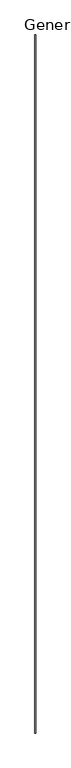
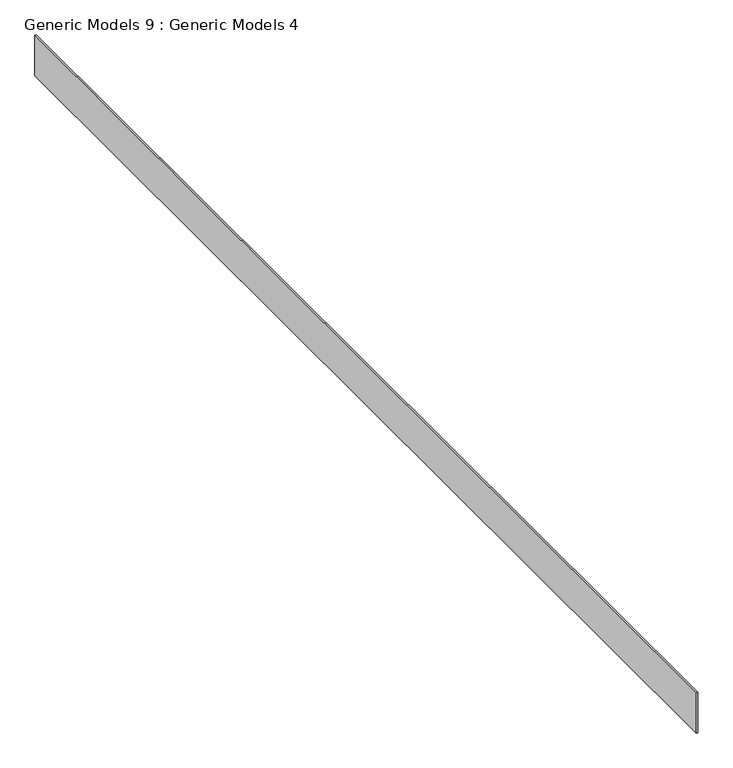
"""IFC4 building model written with IfcOpenShell, lengths in millimetres: proxy geometry, Generic Models 9 : Generic Models 4."""

from ifc_helpers import new_model, si_unit, frame, origin, place, context, project, spatial, polyline, outline, extrude, source, transform, mapped, element, save


def generic_models_9_generic_models_4_ab00bce6(model_context):
    return source(origin(), model_context, "Body", "SweptSolid", [
        extrude(outline(polyline([(8436.6513263, -6864.9230338), (8417.6013263, -6864.9230338), (8417.6013263, 11778.6769662), (8436.6513263, 11778.6769662), (8436.6513263, -6864.9230338)])), frame((0.0, 0.0, 126372.2280968), z_axis=(0.0, 0.0, 1.0), x_axis=(1.0, 0.0, 0.0)), (0.0, 0.0, 1.0), 698.1402691),
    ])


if __name__ == "__main__":
    model = new_model("IFC4")
    model_context = context("Model", 3, world=origin())
    ifc_project = project(units=[si_unit("LENGTHUNIT", "METRE", prefix="MILLI")], contexts=[model_context])
    site = spatial("IfcSite", under=ifc_project)
    building = spatial("IfcBuilding", under=site)
    placement = place(None, origin())
    generic_models_9_generic_models_4_shape = generic_models_9_generic_models_4_ab00bce6(model_context)
    element("IfcBuildingElementProxy", 1, Name="Generic Models 9 : Generic Models 4", ObjectType="Generic Models 9 : Generic Models 4", at=placement, inside=building, context=model_context, shape_type="MappedRepresentation", body=[
        mapped(generic_models_9_generic_models_4_shape, transform((0.0, 0.0, 0.0), x_axis=(1.0, 0.0, 0.0), y_axis=(0.0, 1.0, 0.0), z_axis=(0.0, 0.0, 1.0))),
    ])
    save(model, "model.ifc")

# Revit data of these elements
# Element 1 (IfcBuildingElementProxy, "Generic Models 9 : Generic Models 4")
#   Materials on its faces: "_CDX PLYWOOD - SEE STRUCT DWGs"
# Materials
#   "_CDX PLYWOOD - SEE STRUCT DWGs": class "Generic", colour RGB 98 75 74, transparency 0, Cost = 0
